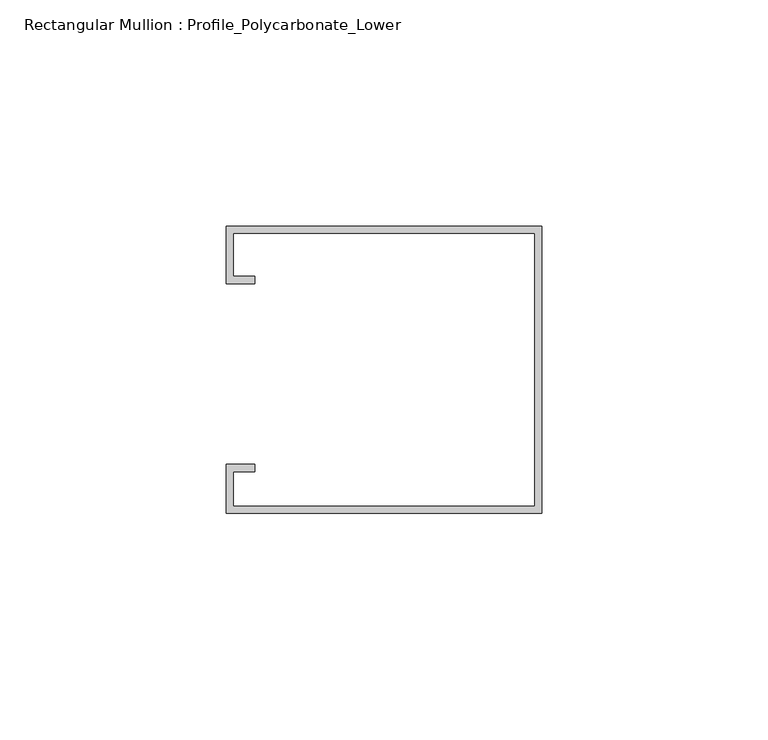
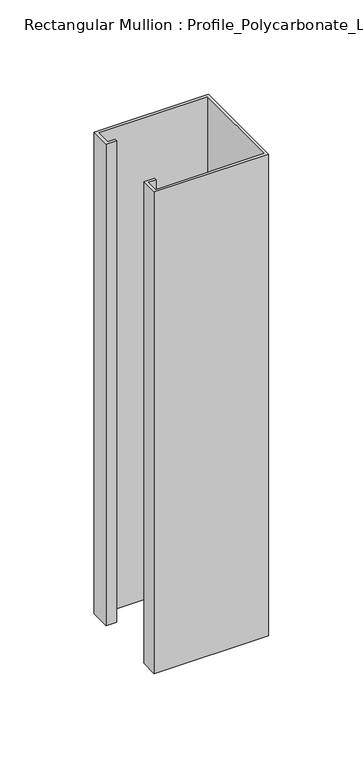
"""IFC4 building model written with IfcOpenShell, lengths in millimetres: member geometry, Rectangular Mullion : Profile_Polycarbonate_Lower."""

import ifcopenshell
import ifcopenshell.guid

model = None  # the IFC model being written
_history = None  # IfcOwnerHistory: only IFC2X3 demands one
_inside = {}  # id of a spatial element -> (the spatial element, [elements in it])
_under = {}  # id of a project, library or spatial element -> (it, [spatial elements below it])
_declared = {}  # id of a project -> (the project, [libraries it declares])
_typed = {}  # id of a type object -> (the type object, [elements of that type])
_made_of = {}  # id of a material, layer set ... -> (it, [elements and type objects made of it])


def new_model(schema):
    """Start an empty IFC model of exactly this schema.

    Asked for "IFC4X3", IfcOpenShell would pick the latest addendum, in which some entities
    have other attributes; the version numbers below select the first issue.
    IFC2X3 requires an IfcOwnerHistory on every rooted entity: one is made here for all.
    """
    global model, _history
    if schema == "IFC4X3":
        model = ifcopenshell.file(schema_version=(4, 3, 0, 0))
    else:
        model = ifcopenshell.file(schema=schema)
    _inside.clear()
    _under.clear()
    _declared.clear()
    _typed.clear()
    _made_of.clear()
    _history = None
    if model.schema == "IFC2X3":
        org = make("IfcOrganization", Name="unknown")
        user = make(
            "IfcPersonAndOrganization",
            ThePerson=make("IfcPerson", FamilyName="unknown"),
            TheOrganization=org,
        )
        app = make(
            "IfcApplication",
            ApplicationDeveloper=org,
            Version="unknown",
            ApplicationFullName="unknown",
            ApplicationIdentifier="unknown",
        )
        _history = make(
            "IfcOwnerHistory",
            OwningUser=user,
            OwningApplication=app,
            ChangeAction="ADDED",
            CreationDate=0,
        )
    return model


def make(cls, **values):
    """One entity of the class cls with the attributes given. An attribute that is None is left unset."""
    return model.create_entity(
        cls, **{name: value for name, value in values.items() if value is not None}
    )


def rooted(cls, **values):
    """An entity with a GlobalId (a new one), such as an element, a storey or a relation."""
    return make(cls, GlobalId=ifcopenshell.guid.new(), OwnerHistory=_history, **values)


def si_unit(unit_type, name, prefix=None):
    """IfcSIUnit, for example si_unit("LENGTHUNIT", "METRE", prefix="MILLI")."""
    return make("IfcSIUnit", UnitType=unit_type, Prefix=prefix, Name=name)


def assignment(units):
    """IfcUnitAssignment: the units of a project."""
    return None if units is None else make("IfcUnitAssignment", Units=units)


def point(xyz):
    """IfcCartesianPoint."""
    return None if xyz is None else make("IfcCartesianPoint", Coordinates=xyz)


def direction(xyz):
    """IfcDirection."""
    return None if xyz is None else make("IfcDirection", DirectionRatios=xyz)


def frame(location, z_axis=None, x_axis=None):
    """IfcAxis2Placement3D, a coordinate frame: its origin and axes. An axis left out is left unset."""
    return make(
        "IfcAxis2Placement3D",
        Location=point(location),
        Axis=direction(z_axis),
        RefDirection=direction(x_axis),
    )


def origin():
    """The frame at (0, 0, 0) with its axes left unset."""
    return frame((0.0, 0.0, 0.0))


def place(relative_to, where):
    """IfcLocalPlacement: puts the frame where relative to a parent placement (None: the world)."""
    return make(
        "IfcLocalPlacement", PlacementRelTo=relative_to, RelativePlacement=where
    )


def context(
    kind, dimensions, precision=None, world=None, true_north=None, identifier=None
):
    """IfcGeometricRepresentationContext, for example the 3D "Model" context."""
    return make(
        "IfcGeometricRepresentationContext",
        ContextIdentifier=identifier,
        ContextType=kind,
        CoordinateSpaceDimension=dimensions,
        Precision=precision,
        WorldCoordinateSystem=world,
        TrueNorth=true_north,
    )


def project(units=None, contexts=None):
    """IfcProject with its units and contexts."""
    return rooted(
        "IfcProject",
        Name="project",
        RepresentationContexts=contexts,
        UnitsInContext=assignment(units),
    )


def spatial(cls, under=None, at=None, **own):
    """A site, building, storey or space (cls), placed at a placement, below another one or the project."""
    s = rooted(cls, ObjectPlacement=at, **own)
    if under is not None:
        _under.setdefault(under.id(), (under, []))[1].append(s)
    return s


def polyline(points):
    """IfcPolyline through the points."""
    return make("IfcPolyline", Points=[point(p) for p in points])


def outline(outer, holes=None, kind="AREA"):
    """IfcArbitraryClosedProfileDef: a profile drawn as a closed curve; with holes, ...WithVoids."""
    if holes is None:
        return make("IfcArbitraryClosedProfileDef", ProfileType=kind, OuterCurve=outer)
    return make(
        "IfcArbitraryProfileDefWithVoids",
        ProfileType=kind,
        OuterCurve=outer,
        InnerCurves=holes,
    )


def extrude(swept, where, along, depth):
    """IfcExtrudedAreaSolid: the profile swept, set in the frame where, extruded along a direction by depth."""
    return make(
        "IfcExtrudedAreaSolid",
        SweptArea=swept,
        Position=where,
        ExtrudedDirection=direction(along),
        Depth=depth,
    )


def shape(context_of_items, identifier, shape_type, items):
    """IfcShapeRepresentation: the items that make up one representation, for example the "Body"."""
    return make(
        "IfcShapeRepresentation",
        ContextOfItems=context_of_items,
        RepresentationIdentifier=identifier,
        RepresentationType=shape_type,
        Items=items,
    )


def source(mapping_origin, context_of_items, identifier, shape_type, items):
    """IfcRepresentationMap: a shape defined once, which mapped items show again and again."""
    return make(
        "IfcRepresentationMap",
        MappingOrigin=mapping_origin,
        MappedRepresentation=shape(context_of_items, identifier, shape_type, items),
    )


def transform(
    local_origin,
    x_axis=None,
    y_axis=None,
    z_axis=None,
    scale=None,
    scale2=None,
    scale3=None,
    uniform=True,
):
    """IfcCartesianTransformationOperator3D, or its non-uniform kind. x_axis, y_axis, z_axis: its Axis1, 2, 3."""
    if uniform:
        return make(
            "IfcCartesianTransformationOperator3D",
            Axis1=direction(x_axis),
            Axis2=direction(y_axis),
            LocalOrigin=point(local_origin),
            Scale=scale,
            Axis3=direction(z_axis),
        )
    return make(
        "IfcCartesianTransformationOperator3DnonUniform",
        Axis1=direction(x_axis),
        Axis2=direction(y_axis),
        LocalOrigin=point(local_origin),
        Scale=scale,
        Axis3=direction(z_axis),
        Scale2=scale2,
        Scale3=scale3,
    )


def mapped(mapping_source, mapping_target):
    """IfcMappedItem: shows the shape of a source again, moved by a transform."""
    return make(
        "IfcMappedItem", MappingSource=mapping_source, MappingTarget=mapping_target
    )


def made_of(thing, what):
    """Note that an element or type object is made of a material, layer set ...; save() writes the relation."""
    if what is not None:
        _made_of.setdefault(what.id(), (what, []))[1].append(thing)
    return thing


def element(
    cls,
    number,
    at=None,
    inside=None,
    cuts=None,
    type_object=None,
    material=None,
    context=None,
    identifier="Body",
    shape_type=None,
    held_by="IfcProductDefinitionShape",
    body=None,
    shapes=None,
    **own,
):
    """One element of the class cls, such as IfcWall. Its Tag is "e" and its number.

    at: its placement. inside: the storey or other place that contains it. cuts: it is an
    opening in that element (IfcRelVoidsElement). A single representation is given by context,
    identifier, shape_type and body (its items); several are given by shapes. held_by: the class
    of the entity that holds the representations. save() writes the other relations.
    """
    e = rooted(cls, Tag="e%d" % number, ObjectPlacement=at, **own)
    if body is not None:
        shapes = [shape(context, identifier, shape_type, body)]
    if shapes is not None:
        e.Representation = make(held_by, Representations=shapes)
    if inside is not None:
        _inside.setdefault(inside.id(), (inside, []))[1].append(e)
    if cuts is not None:
        rooted(
            "IfcRelVoidsElement", RelatingBuildingElement=cuts, RelatedOpeningElement=e
        )
    if type_object is not None:
        _typed.setdefault(type_object.id(), (type_object, []))[1].append(e)
    return made_of(e, material)


def aggregate(whole, parts):
    """IfcRelAggregates: a whole, such as a stair, and the parts it consists of."""
    return rooted("IfcRelAggregates", RelatingObject=whole, RelatedObjects=parts)


def save(model, path):
    """Write the relations noted so far, then the file.

    IfcRelAggregates (storeys below a building ...), IfcRelContainedInSpatialStructure (elements
    in a storey), IfcRelDefinesByType, IfcRelAssociatesMaterial and IfcRelDeclares: one each for
    every whole, place, type object, material and project.
    """
    for whole, parts in _under.values():
        aggregate(whole, parts)
    for where, things in _inside.values():
        rooted(
            "IfcRelContainedInSpatialStructure",
            RelatedElements=things,
            RelatingStructure=where,
        )
    for kind, things in _typed.values():
        rooted("IfcRelDefinesByType", RelatedObjects=things, RelatingType=kind)
    for what, things in _made_of.values():
        rooted("IfcRelAssociatesMaterial", RelatedObjects=things, RelatingMaterial=what)
    for by, libraries in _declared.values():
        rooted("IfcRelDeclares", RelatingContext=by, RelatedDefinitions=libraries)
    model.write(path)


def rectangular_mullion_profile_polycarbonate_lower_2fe27bd3(model_context):
    return source(origin(), model_context, "Body", "SweptSolid", [
        extrude(outline(polyline([(0.0, 32.7), (0.0, -30.8), (-69.85, -30.8), (-69.85, -20.0), (-63.5, -20.0), (-63.5, -21.5875), (-68.2625, -21.5875), (-68.2625, -29.2125), (-1.5875, -29.2125), (-1.5875, 31.1125), (-68.2625, 31.1125), (-68.2625, 21.5875), (-63.5, 21.5875), (-63.5, 20.0), (-69.85, 20.0), (-69.85, 32.7), (0.0, 32.7)])), frame((0.0, 0.0, -311.15), z_axis=(0.0, 0.0, 1.0), x_axis=(1.0, 0.0, 0.0)), (0.0, 0.0, 1.0), 311.15),
    ])


if __name__ == "__main__":
    model = new_model("IFC4")
    model_context = context("Model", 3, world=origin())
    ifc_project = project(units=[si_unit("LENGTHUNIT", "METRE", prefix="MILLI")], contexts=[model_context])
    site = spatial("IfcSite", under=ifc_project)
    building = spatial("IfcBuilding", under=site)
    placement = place(None, origin())
    rectangular_mullion_profile_polycarbonate_lower_shape = rectangular_mullion_profile_polycarbonate_lower_2fe27bd3(model_context)
    element("IfcMember", 1, ObjectType="Rectangular Mullion : Profile_Polycarbonate_Lower", at=placement, inside=building, context=model_context, shape_type="MappedRepresentation", body=[
        mapped(rectangular_mullion_profile_polycarbonate_lower_shape, transform((0.0, 0.0, 0.0), x_axis=(1.0, 0.0, 0.0), y_axis=(0.0, 1.0, 0.0), z_axis=(0.0, 0.0, 1.0))),
    ])
    save(model, "model.ifc")

# Revit data of these elements
# Type "Rectangular Mullion : Profile_Polycarbonate_Lower"
#   built-in parameter 1007322 = 0.208333 (stored number, unit not read)
#   built-in parameter 1007321 = 0 (stored number, unit not read)
#   built-in parameter 1007320 = 0.00520833 (stored number, unit not read)
# Element 1 (IfcMember, "Rectangular Mullion : Profile_Polycarbonate_Lower")
#   Materials on its faces: "GALVANIZED UNISTRUT P5500, 1 5/8\" X 2 7/16\" OR ALUM. CHANNEL"
# Materials
#   "GALVANIZED UNISTRUT P5500, 1 5/8\" X 2 7/16\" OR ALUM. CHANNEL": class "Metal", colour RGB 244 244 244, transparency 0, Description = "Aluminum 6061", Cost = 0
